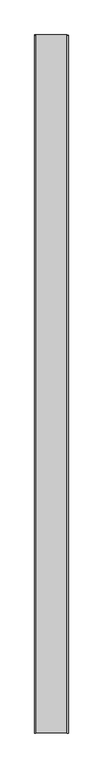
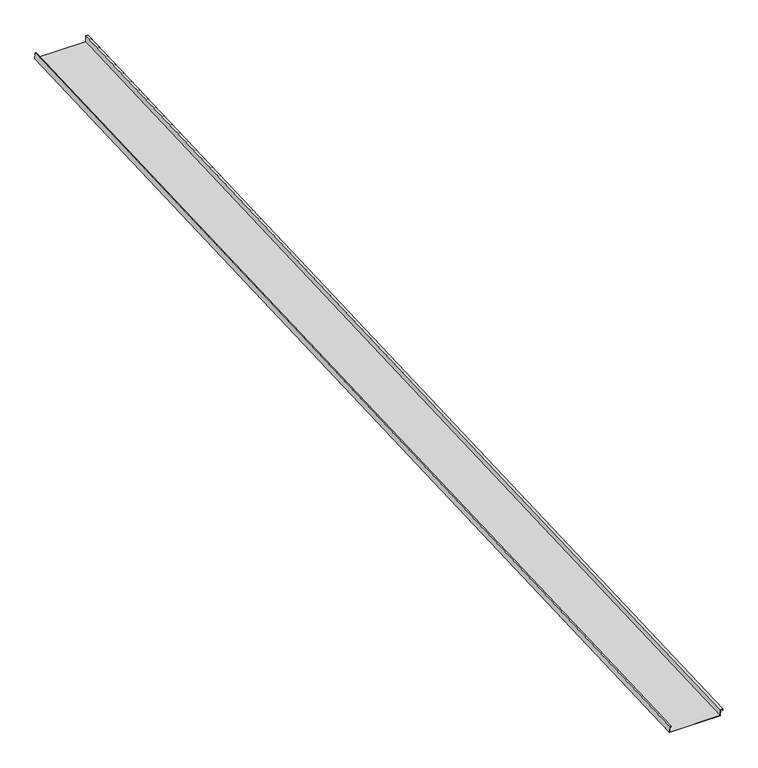
"""IFC4 building model written with IfcOpenShell, lengths in millimetres: proxy geometry, Generic Models 2:Generic Models 2:310765:Generic Models 2:310765 : Generic Models 2:Generic Models 2:310765:200 : Generic Models 2:Generic Models 2:310765:Generic Models 2:310765 : Generic Models 2:Generic Models 2:310765:300385."""

from ifc_helpers import new_model, si_unit, frame, origin, place, context, project, spatial, polyline, outline, extrude, source, transform, mapped, element, save


def generic_models_ad1a354e(model_context):
    return source(origin(), model_context, "Body", "SweptSolid", [
        extrude(outline(polyline([(50.8000001, 0.0), (50.8000001, 14.2875), (41.275, 14.2875), (41.275, 15.875), (52.3875, 15.875), (52.3875, -1.5875), (1.5875, -1.5875), (1.5875, -404.8125), (47.625, -404.8125), (47.625, -396.875), (39.6875001, -396.875), (39.6875001, -395.2875), (49.2125, -395.2875), (49.2125, -406.4), (0.0, -406.4), (0.0, 0.0), (50.8000001, 0.0)])), frame((579984.8218144, -580678.4204475, 3889.8616527), z_axis=(0.0, 0.9991330730923567, 0.04163054471206783), x_axis=(0.0, -0.04163054471206783, 0.9991330730923567)), (0.0, 0.0, 1.0), 8776.7038972),
    ])


if __name__ == "__main__":
    model = new_model("IFC4")
    model_context = context("Model", 3, world=origin())
    ifc_project = project(units=[si_unit("LENGTHUNIT", "METRE", prefix="MILLI")], contexts=[model_context])
    site = spatial("IfcSite", under=ifc_project)
    building = spatial("IfcBuilding", under=site)
    placement = place(None, origin())
    generic_models_shape = generic_models_ad1a354e(model_context)
    element("IfcBuildingElementProxy", 1, Name="Generic Models 2:Generic Models 2:310765:Generic Models 2:310765 : Generic Models 2:Generic Models 2:310765:200 : Generic Models 2:Generic Models 2:310765:Generic Models 2:310765 : Generic Models 2:Generic Models 2:310765:300385", ObjectType="Generic Models 2:Generic Models 2:310765:Generic Models 2:310765 : Generic Models 2:Generic Models 2:310765:200 : Generic Models 2:Generic Models 2:310765:Generic Models 2:310765 : Generic Models 2:Generic Models 2:310765:300385", at=placement, inside=building, context=model_context, shape_type="MappedRepresentation", body=[
        mapped(generic_models_shape, transform((0.0, 0.0, 0.0), x_axis=(1.0, 0.0, 0.0), y_axis=(0.0, 1.0, 0.0), z_axis=(0.0, 0.0, 1.0))),
    ])
    save(model, "model.ifc")

# Revit data of these elements
# Type "Generic Models 2:Generic Models 2:310765:Generic Models 2:310765 : Generic Models 2:Generic Models 2:310765:200 : Generic Models 2:Generic Models 2:310765:Generic Models 2:310765 : Generic Models 2:Generic Models 2:310765:300385"
#   NameOverride = "Generic Models 2:Generic Models 2:310765:Generic Models 2:310765 : Generic Models 2:Generic Models 2:310765:300385"
#   ObjectTypeOverride = "Generic Models 2:310765 : Generic Models 2:Generic Models 2:310765"
#   Reference = "Generic Models 2"
#   Tag = "300385"
# Element 1 (IfcBuildingElementProxy, "Generic Models 2:Generic Models 2:310765:Generic Models 2:310765 : Generic Models 2:Generic Models 2:310765:200 : Generic Models 2:Generic Models 2:310765:Generic Models 2:310765 : Generic Models 2:Generic Models 2:310765:300385")
#   Materials on its faces: "STRUCTURAL STANDING SEAM SHEET METAL ROOFING - BATTENLOK - COLOR T.B.D."
# Materials
#   "STRUCTURAL STANDING SEAM SHEET METAL ROOFING - BATTENLOK - COLOR T.B.D.": class "Generic", colour RGB 120 120 120, transparency 0, Cost = 0
